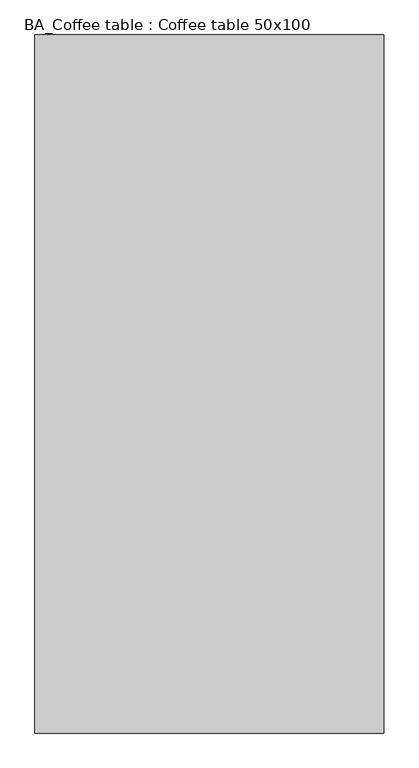
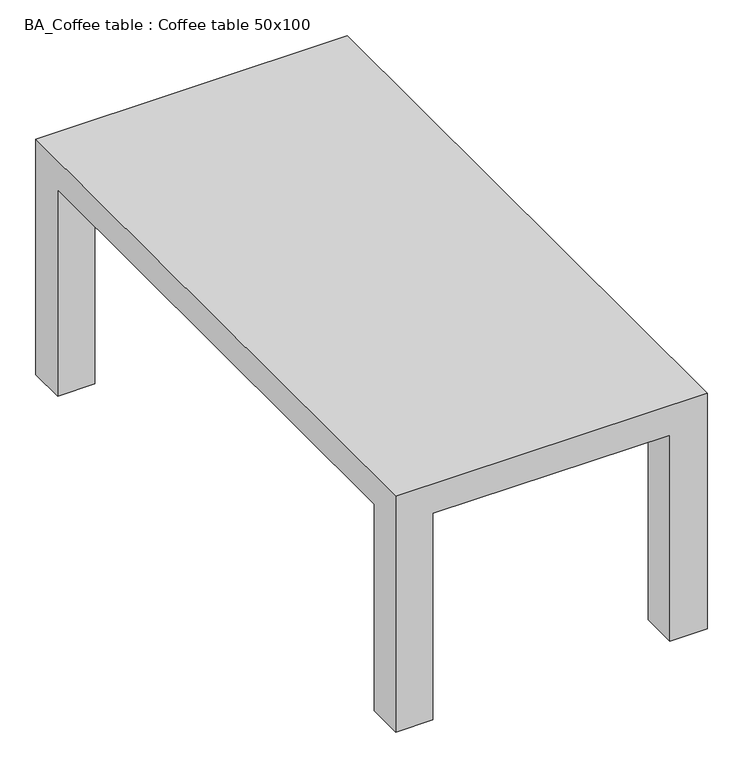
"""IFC4 building model written with IfcOpenShell, lengths in millimetres: furniture geometry, BA_Coffee table : Coffee table 50x100."""

from ifc_helpers import new_model, si_unit, origin, place, context, project, spatial, faceted_brep, source, transform, mapped, element, save


def ba_coffee_table_coffee_table_50x100_c3c5c219(model_context):
    return source(origin(), model_context, "Body", "Brep", [
        faceted_brep([(-190.0, -440.0, 0.0), (-190.0, -500.0, 0.0), (-250.0, -500.0, 0.0), (-250.0, -440.0, 0.0), (-250.0, -440.0, 350.0), (-190.0, -440.0, 350.0), (-250.0, -500.0, 400.0), (-250.0, 500.0, 400.0), (-250.0, 500.0, 0.0), (-250.0, 440.0, 0.0), (-250.0, 440.0, 350.0), (-190.0, -500.0, 350.0), (190.0, -500.0, 350.0), (190.0, -500.0, 0.0), (250.0, -500.0, 0.0), (250.0, -500.0, 400.0), (250.0, 500.0, 400.0), (-190.0, 440.0, 350.0), (-190.0, 500.0, 350.0), (190.0, 500.0, 350.0), (190.0, 440.0, 350.0), (250.0, 440.0, 350.0), (250.0, -440.0, 350.0), (190.0, -440.0, 350.0), (250.0, 500.0, 0.0), (190.0, 500.0, 0.0), (-190.0, 500.0, 0.0), (250.0, -440.0, 0.0), (250.0, 440.0, 0.0), (190.0, -440.0, 0.0), (-190.0, 440.0, 0.0), (190.0, 440.0, 0.0)], [[[0, 1, 2, 3]], [[0, 3, 4, 5]], [[3, 2, 6, 7, 8, 9, 10, 4]], [[2, 1, 11, 12, 13, 14, 15, 6]], [[1, 0, 5, 11]], [[16, 7, 6, 15]], [[5, 4, 10, 17, 18, 19, 20, 21, 22, 23, 12, 11]], [[7, 16, 24, 25, 19, 18, 26, 8]], [[24, 16, 15, 14, 27, 22, 21, 28]], [[27, 14, 13, 29]], [[27, 29, 23, 22]], [[29, 13, 12, 23]], [[26, 30, 9, 8]], [[9, 30, 17, 10]], [[30, 26, 18, 17]], [[24, 28, 31, 25]], [[25, 31, 20, 19]], [[31, 28, 21, 20]]]),
    ])


if __name__ == "__main__":
    model = new_model("IFC4")
    model_context = context("Model", 3, world=origin())
    ifc_project = project(units=[si_unit("LENGTHUNIT", "METRE", prefix="MILLI")], contexts=[model_context])
    site = spatial("IfcSite", under=ifc_project)
    building = spatial("IfcBuilding", under=site)
    placement = place(None, origin())
    ba_coffee_table_coffee_table_50x100_shape = ba_coffee_table_coffee_table_50x100_c3c5c219(model_context)
    element("IfcFurniture", 1, ObjectType="BA_Coffee table : Coffee table 50x100", at=placement, inside=building, context=model_context, shape_type="MappedRepresentation", body=[
        mapped(ba_coffee_table_coffee_table_50x100_shape, transform((0.0, 0.0, 0.0), x_axis=(1.0, 0.0, 0.0), y_axis=(0.0, 1.0, 0.0), z_axis=(0.0, 0.0, 1.0))),
    ])
    save(model, "model.ifc")

# Revit data of these elements
# Type "BA_Coffee table : Coffee table 50x100"
#   height = 400 mm
#   width = 500 mm
#   length = 1000 mm
#   Default Elevation = 0
# Element 1 (IfcFurniture, "BA_Coffee table : Coffee table 50x100")
#   Materials on its faces: "Default"
# Materials
#   "Default": class "Generic", colour RGB 255 255 255, transparency 0, Cost = 0
